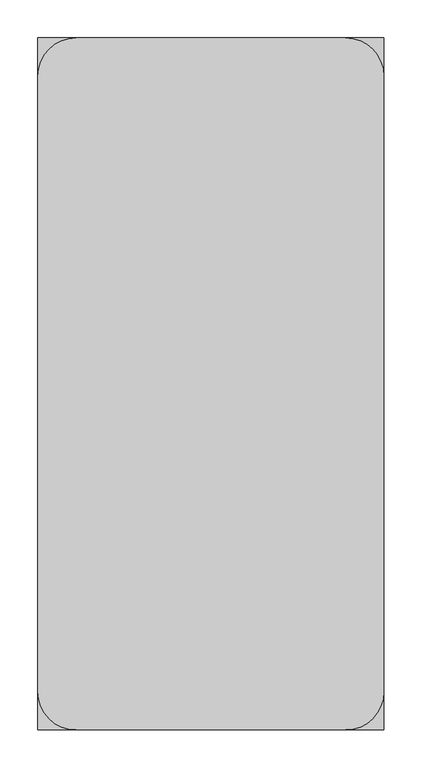
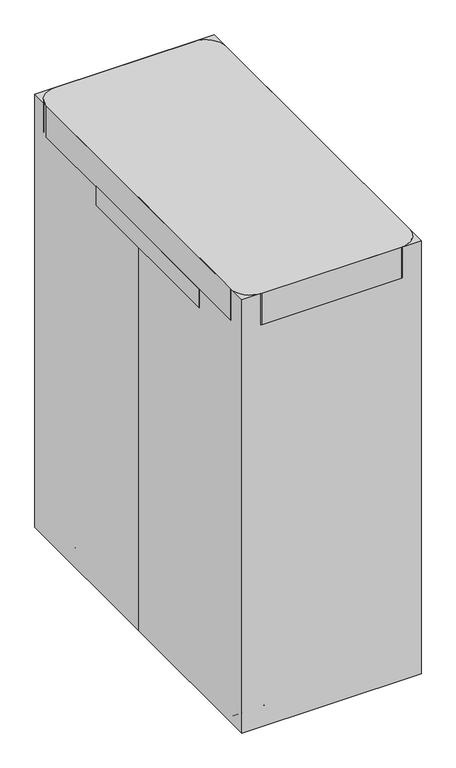
"""IFC4 building model written with IfcOpenShell, lengths in millimetres: proxy geometry, M7040 - Table, Overbed : M7040 - Table, Overbed."""

import ifcopenshell
import ifcopenshell.guid

model = None  # the IFC model being written
_history = None  # IfcOwnerHistory: only IFC2X3 demands one
_inside = {}  # id of a spatial element -> (the spatial element, [elements in it])
_under = {}  # id of a project, library or spatial element -> (it, [spatial elements below it])
_declared = {}  # id of a project -> (the project, [libraries it declares])
_typed = {}  # id of a type object -> (the type object, [elements of that type])
_made_of = {}  # id of a material, layer set ... -> (it, [elements and type objects made of it])


def new_model(schema):
    """Start an empty IFC model of exactly this schema.

    Asked for "IFC4X3", IfcOpenShell would pick the latest addendum, in which some entities
    have other attributes; the version numbers below select the first issue.
    IFC2X3 requires an IfcOwnerHistory on every rooted entity: one is made here for all.
    """
    global model, _history
    if schema == "IFC4X3":
        model = ifcopenshell.file(schema_version=(4, 3, 0, 0))
    else:
        model = ifcopenshell.file(schema=schema)
    _inside.clear()
    _under.clear()
    _declared.clear()
    _typed.clear()
    _made_of.clear()
    _history = None
    if model.schema == "IFC2X3":
        org = make("IfcOrganization", Name="unknown")
        user = make(
            "IfcPersonAndOrganization",
            ThePerson=make("IfcPerson", FamilyName="unknown"),
            TheOrganization=org,
        )
        app = make(
            "IfcApplication",
            ApplicationDeveloper=org,
            Version="unknown",
            ApplicationFullName="unknown",
            ApplicationIdentifier="unknown",
        )
        _history = make(
            "IfcOwnerHistory",
            OwningUser=user,
            OwningApplication=app,
            ChangeAction="ADDED",
            CreationDate=0,
        )
    return model


def make(cls, **values):
    """One entity of the class cls with the attributes given. An attribute that is None is left unset."""
    return model.create_entity(
        cls, **{name: value for name, value in values.items() if value is not None}
    )


def rooted(cls, **values):
    """An entity with a GlobalId (a new one), such as an element, a storey or a relation."""
    return make(cls, GlobalId=ifcopenshell.guid.new(), OwnerHistory=_history, **values)


def si_unit(unit_type, name, prefix=None):
    """IfcSIUnit, for example si_unit("LENGTHUNIT", "METRE", prefix="MILLI")."""
    return make("IfcSIUnit", UnitType=unit_type, Prefix=prefix, Name=name)


def assignment(units):
    """IfcUnitAssignment: the units of a project."""
    return None if units is None else make("IfcUnitAssignment", Units=units)


def point(xyz):
    """IfcCartesianPoint."""
    return None if xyz is None else make("IfcCartesianPoint", Coordinates=xyz)


def direction(xyz):
    """IfcDirection."""
    return None if xyz is None else make("IfcDirection", DirectionRatios=xyz)


def frame(location, z_axis=None, x_axis=None):
    """IfcAxis2Placement3D, a coordinate frame: its origin and axes. An axis left out is left unset."""
    return make(
        "IfcAxis2Placement3D",
        Location=point(location),
        Axis=direction(z_axis),
        RefDirection=direction(x_axis),
    )


def frame_2d(location, x_axis=None):
    """IfcAxis2Placement2D, a coordinate frame in the plane: its origin and x axis."""
    return make(
        "IfcAxis2Placement2D", Location=point(location), RefDirection=direction(x_axis)
    )


def origin():
    """The frame at (0, 0, 0) with its axes left unset."""
    return frame((0.0, 0.0, 0.0))


def origin_with_axes():
    """The frame at (0, 0, 0) with the z axis (0, 0, 1) and the x axis (1, 0, 0) written out."""
    return frame((0.0, 0.0, 0.0), z_axis=(0.0, 0.0, 1.0), x_axis=(1.0, 0.0, 0.0))


def place(relative_to, where):
    """IfcLocalPlacement: puts the frame where relative to a parent placement (None: the world)."""
    return make(
        "IfcLocalPlacement", PlacementRelTo=relative_to, RelativePlacement=where
    )


def context(
    kind, dimensions, precision=None, world=None, true_north=None, identifier=None
):
    """IfcGeometricRepresentationContext, for example the 3D "Model" context."""
    return make(
        "IfcGeometricRepresentationContext",
        ContextIdentifier=identifier,
        ContextType=kind,
        CoordinateSpaceDimension=dimensions,
        Precision=precision,
        WorldCoordinateSystem=world,
        TrueNorth=true_north,
    )


def project(units=None, contexts=None):
    """IfcProject with its units and contexts."""
    return rooted(
        "IfcProject",
        Name="project",
        RepresentationContexts=contexts,
        UnitsInContext=assignment(units),
    )


def spatial(cls, under=None, at=None, **own):
    """A site, building, storey or space (cls), placed at a placement, below another one or the project."""
    s = rooted(cls, ObjectPlacement=at, **own)
    if under is not None:
        _under.setdefault(under.id(), (under, []))[1].append(s)
    return s


def polyline(points):
    """IfcPolyline through the points."""
    return make("IfcPolyline", Points=[point(p) for p in points])


def circle_curve(where, radius):
    """IfcCircle in the frame where."""
    return make("IfcCircle", Position=where, Radius=radius)


def trimmed(basis, trim1, trim2, sense, master):
    """IfcTrimmedCurve: the piece of a basis curve between two trims."""
    return make(
        "IfcTrimmedCurve",
        BasisCurve=basis,
        Trim1=trim1,
        Trim2=trim2,
        SenseAgreement=sense,
        MasterRepresentation=master,
    )


def segment(curve, same_sense, transition):
    """IfcCompositeCurveSegment."""
    return make(
        "IfcCompositeCurveSegment",
        Transition=transition,
        SameSense=same_sense,
        ParentCurve=curve,
    )


def composite_curve(segments, self_intersect=None):
    """IfcCompositeCurve: segments joined end to end."""
    return make("IfcCompositeCurve", Segments=segments, SelfIntersect=self_intersect)


def outline(outer, holes=None, kind="AREA"):
    """IfcArbitraryClosedProfileDef: a profile drawn as a closed curve; with holes, ...WithVoids."""
    if holes is None:
        return make("IfcArbitraryClosedProfileDef", ProfileType=kind, OuterCurve=outer)
    return make(
        "IfcArbitraryProfileDefWithVoids",
        ProfileType=kind,
        OuterCurve=outer,
        InnerCurves=holes,
    )


def extrude(swept, where, along, depth):
    """IfcExtrudedAreaSolid: the profile swept, set in the frame where, extruded along a direction by depth."""
    return make(
        "IfcExtrudedAreaSolid",
        SweptArea=swept,
        Position=where,
        ExtrudedDirection=direction(along),
        Depth=depth,
    )


def shape(context_of_items, identifier, shape_type, items):
    """IfcShapeRepresentation: the items that make up one representation, for example the "Body"."""
    return make(
        "IfcShapeRepresentation",
        ContextOfItems=context_of_items,
        RepresentationIdentifier=identifier,
        RepresentationType=shape_type,
        Items=items,
    )


def source(mapping_origin, context_of_items, identifier, shape_type, items):
    """IfcRepresentationMap: a shape defined once, which mapped items show again and again."""
    return make(
        "IfcRepresentationMap",
        MappingOrigin=mapping_origin,
        MappedRepresentation=shape(context_of_items, identifier, shape_type, items),
    )


def transform(
    local_origin,
    x_axis=None,
    y_axis=None,
    z_axis=None,
    scale=None,
    scale2=None,
    scale3=None,
    uniform=True,
):
    """IfcCartesianTransformationOperator3D, or its non-uniform kind. x_axis, y_axis, z_axis: its Axis1, 2, 3."""
    if uniform:
        return make(
            "IfcCartesianTransformationOperator3D",
            Axis1=direction(x_axis),
            Axis2=direction(y_axis),
            LocalOrigin=point(local_origin),
            Scale=scale,
            Axis3=direction(z_axis),
        )
    return make(
        "IfcCartesianTransformationOperator3DnonUniform",
        Axis1=direction(x_axis),
        Axis2=direction(y_axis),
        LocalOrigin=point(local_origin),
        Scale=scale,
        Axis3=direction(z_axis),
        Scale2=scale2,
        Scale3=scale3,
    )


def mapped(mapping_source, mapping_target):
    """IfcMappedItem: shows the shape of a source again, moved by a transform."""
    return make(
        "IfcMappedItem", MappingSource=mapping_source, MappingTarget=mapping_target
    )


def made_of(thing, what):
    """Note that an element or type object is made of a material, layer set ...; save() writes the relation."""
    if what is not None:
        _made_of.setdefault(what.id(), (what, []))[1].append(thing)
    return thing


def element(
    cls,
    number,
    at=None,
    inside=None,
    cuts=None,
    type_object=None,
    material=None,
    context=None,
    identifier="Body",
    shape_type=None,
    held_by="IfcProductDefinitionShape",
    body=None,
    shapes=None,
    **own,
):
    """One element of the class cls, such as IfcWall. Its Tag is "e" and its number.

    at: its placement. inside: the storey or other place that contains it. cuts: it is an
    opening in that element (IfcRelVoidsElement). A single representation is given by context,
    identifier, shape_type and body (its items); several are given by shapes. held_by: the class
    of the entity that holds the representations. save() writes the other relations.
    """
    e = rooted(cls, Tag="e%d" % number, ObjectPlacement=at, **own)
    if body is not None:
        shapes = [shape(context, identifier, shape_type, body)]
    if shapes is not None:
        e.Representation = make(held_by, Representations=shapes)
    if inside is not None:
        _inside.setdefault(inside.id(), (inside, []))[1].append(e)
    if cuts is not None:
        rooted(
            "IfcRelVoidsElement", RelatingBuildingElement=cuts, RelatedOpeningElement=e
        )
    if type_object is not None:
        _typed.setdefault(type_object.id(), (type_object, []))[1].append(e)
    return made_of(e, material)


def aggregate(whole, parts):
    """IfcRelAggregates: a whole, such as a stair, and the parts it consists of."""
    return rooted("IfcRelAggregates", RelatingObject=whole, RelatedObjects=parts)


def save(model, path):
    """Write the relations noted so far, then the file.

    IfcRelAggregates (storeys below a building ...), IfcRelContainedInSpatialStructure (elements
    in a storey), IfcRelDefinesByType, IfcRelAssociatesMaterial and IfcRelDeclares: one each for
    every whole, place, type object, material and project.
    """
    for whole, parts in _under.values():
        aggregate(whole, parts)
    for where, things in _inside.values():
        rooted(
            "IfcRelContainedInSpatialStructure",
            RelatedElements=things,
            RelatingStructure=where,
        )
    for kind, things in _typed.values():
        rooted("IfcRelDefinesByType", RelatedObjects=things, RelatingType=kind)
    for what, things in _made_of.values():
        rooted("IfcRelAssociatesMaterial", RelatedObjects=things, RelatingMaterial=what)
    for by, libraries in _declared.values():
        rooted("IfcRelDeclares", RelatingContext=by, RelatedDefinitions=libraries)
    model.write(path)


def specialty_equipment_190c61b0(model_context):
    return source(origin(), model_context, "Body", "SweptSolid", [
        extrude(outline(polyline([(228.6, 187.2297287), (228.6, -269.9702713), (-228.6, -269.9702713), (-228.6, 187.2297287), (228.6, 187.2297287)])), frame((0.0, 0.0, 1033.0016667), z_axis=(0.0, 0.0, 1.0), x_axis=(1.0, 0.0, 0.0)), (0.0, 0.0, 1.0), 50.8),
        extrude(outline(polyline([(216.6344082, -319.9060209), (216.6344082, -425.45), (-218.1273098, -425.45), (-218.1273098, -319.9060209), (216.6344082, -319.9060209)])), frame((0.0, 0.0, 127.0), z_axis=(0.0, 0.0, 1.0), x_axis=(1.0, 0.0, 0.0)), (0.0, 0.0, 1.0), 38.1),
        extrude(outline(polyline([(-33.9903673, 310.5535606), (34.925, 310.5535606), (34.925, -319.9060209), (-33.9903673, -319.9060209), (-33.9903673, 310.5535606)])), frame((0.0, 0.0, 127.0), z_axis=(0.0, 0.0, 1.0), x_axis=(1.0, 0.0, 0.0)), (0.0, 0.0, 1.0), 38.1),
        extrude(outline(composite_curve([segment(trimmed(circle_curve(frame_2d((-179.8693101, -389.7056599)), 16.9333333), [point((-196.8026434, -389.7056599))], [point((-162.9359768, -389.7056599))], False, "CARTESIAN"), True, "CONTINUOUS"), segment(trimmed(circle_curve(frame_2d((-179.8693101, -389.7056599)), 16.9333333), [point((-162.9359768, -389.7056599))], [point((-196.8026434, -389.7056599))], False, "CARTESIAN"), True, "CONTINUOUS")], self_intersect=False)), frame((0.0, 0.0, 84.8149176), z_axis=(0.0, 0.0, 1.0), x_axis=(1.0, 0.0, 0.0)), (0.0, 0.0, 1.0), 42.1850824),
        extrude(outline(composite_curve([segment(trimmed(circle_curve(frame_2d((178.8623991, -389.7056599)), 16.9333333), [point((195.7957324, -389.7056599))], [point((161.9290658, -389.7056599))], False, "CARTESIAN"), True, "CONTINUOUS"), segment(trimmed(circle_curve(frame_2d((178.8623991, -389.7056599)), 16.9333333), [point((161.9290658, -389.7056599))], [point((195.7957324, -389.7056599))], False, "CARTESIAN"), True, "CONTINUOUS")], self_intersect=False)), frame((0.0, 0.0, 84.8149176), z_axis=(0.0, 0.0, 1.0), x_axis=(1.0, 0.0, 0.0)), (0.0, 0.0, 1.0), 42.1850824),
        extrude(outline(composite_curve([segment(trimmed(circle_curve(frame_2d((-372.7723265, 50.8)), 50.8), [point((-423.5723265, 50.8))], [point((-321.9723265, 50.8))], False, "CARTESIAN"), True, "CONTINUOUS"), segment(trimmed(circle_curve(frame_2d((-372.7723265, 50.8)), 50.8), [point((-321.9723265, 50.8))], [point((-423.5723265, 50.8))], False, "CARTESIAN"), True, "CONTINUOUS")], self_intersect=False)), frame((140.7840445, 0.0, 0.0), z_axis=(1.0, 0.0, 0.0), x_axis=(0.0, 1.0, 0.0)), (0.0, 0.0, 1.0), 19.05),
        extrude(outline(composite_curve([segment(trimmed(circle_curve(frame_2d((-372.7723265, 50.8)), 50.8), [point((-423.5723265, 50.8))], [point((-321.9723265, 50.8))], False, "CARTESIAN"), True, "CONTINUOUS"), segment(trimmed(circle_curve(frame_2d((-372.7723265, 50.8)), 50.8), [point((-321.9723265, 50.8))], [point((-423.5723265, 50.8))], False, "CARTESIAN"), True, "CONTINUOUS")], self_intersect=False)), frame((197.9340445, 0.0, 0.0), z_axis=(1.0, 0.0, 0.0), x_axis=(0.0, 1.0, 0.0)), (0.0, 0.0, 1.0), 19.05),
        extrude(outline(composite_curve([segment(trimmed(circle_curve(frame_2d((-372.7723265, 50.8)), 33.8666667), [point((-338.9056599, 50.8))], [point((-406.6389932, 50.8))], False, "CARTESIAN"), True, "CONTINUOUS"), segment(trimmed(circle_curve(frame_2d((-372.7723265, 50.8)), 33.8666667), [point((-406.6389932, 50.8))], [point((-338.9056599, 50.8))], False, "CARTESIAN"), True, "CONTINUOUS")], self_intersect=False)), frame((159.8340445, 0.0, 0.0), z_axis=(1.0, 0.0, 0.0), x_axis=(0.0, 1.0, 0.0)), (0.0, 0.0, 1.0), 38.1),
        extrude(outline(composite_curve([segment(trimmed(circle_curve(frame_2d((-372.7723265, 50.8)), 50.8), [point((-423.5723265, 50.8))], [point((-321.9723265, 50.8))], False, "CARTESIAN"), True, "CONTINUOUS"), segment(trimmed(circle_curve(frame_2d((-372.7723265, 50.8)), 50.8), [point((-321.9723265, 50.8))], [point((-423.5723265, 50.8))], False, "CARTESIAN"), True, "CONTINUOUS")], self_intersect=False)), frame((-160.6276735, 0.0, 0.0), z_axis=(1.0, 0.0, 0.0), x_axis=(0.0, 1.0, 0.0)), (0.0, 0.0, 1.0), 19.05),
        extrude(outline(composite_curve([segment(trimmed(circle_curve(frame_2d((-372.7723265, 50.8)), 50.8), [point((-423.5723265, 50.8))], [point((-321.9723265, 50.8))], False, "CARTESIAN"), True, "CONTINUOUS"), segment(trimmed(circle_curve(frame_2d((-372.7723265, 50.8)), 50.8), [point((-321.9723265, 50.8))], [point((-423.5723265, 50.8))], False, "CARTESIAN"), True, "CONTINUOUS")], self_intersect=False)), frame((-217.7776735, 0.0, 0.0), z_axis=(1.0, 0.0, 0.0), x_axis=(0.0, 1.0, 0.0)), (0.0, 0.0, 1.0), 19.05),
        extrude(outline(composite_curve([segment(trimmed(circle_curve(frame_2d((-372.7723265, 50.8)), 33.8666667), [point((-338.9056599, 50.8))], [point((-406.6389932, 50.8))], False, "CARTESIAN"), True, "CONTINUOUS"), segment(trimmed(circle_curve(frame_2d((-372.7723265, 50.8)), 33.8666667), [point((-406.6389932, 50.8))], [point((-338.9056599, 50.8))], False, "CARTESIAN"), True, "CONTINUOUS")], self_intersect=False)), frame((-198.7276735, 0.0, 0.0), z_axis=(1.0, 0.0, 0.0), x_axis=(0.0, 1.0, 0.0)), (0.0, 0.0, 1.0), 38.1),
        extrude(outline(composite_curve([segment(trimmed(circle_curve(frame_2d((-180.2189464, 378.2868939)), 16.9333333), [point((-197.1522798, 378.2868939))], [point((-163.2856131, 378.2868939))], False, "CARTESIAN"), True, "CONTINUOUS"), segment(trimmed(circle_curve(frame_2d((-180.2189464, 378.2868939)), 16.9333333), [point((-163.2856131, 378.2868939))], [point((-197.1522798, 378.2868939))], False, "CARTESIAN"), True, "CONTINUOUS")], self_intersect=False)), frame((0.0, 0.0, 84.8149176), z_axis=(0.0, 0.0, 1.0), x_axis=(1.0, 0.0, 0.0)), (0.0, 0.0, 1.0), 42.1850824),
        extrude(outline(composite_curve([segment(trimmed(circle_curve(frame_2d((178.5127627, 378.2868939)), 16.9333333), [point((195.4460961, 378.2868939))], [point((161.5794294, 378.2868939))], False, "CARTESIAN"), True, "CONTINUOUS"), segment(trimmed(circle_curve(frame_2d((178.5127627, 378.2868939)), 16.9333333), [point((161.5794294, 378.2868939))], [point((195.4460961, 378.2868939))], False, "CARTESIAN"), True, "CONTINUOUS")], self_intersect=False)), frame((0.0, 0.0, 84.8149176), z_axis=(0.0, 0.0, 1.0), x_axis=(1.0, 0.0, 0.0)), (0.0, 0.0, 1.0), 42.1850824),
        extrude(outline(composite_curve([segment(trimmed(circle_curve(frame_2d((361.3535606, 50.8)), 50.8), [point((412.1535606, 50.8))], [point((310.5535606, 50.8))], False, "CARTESIAN"), True, "CONTINUOUS"), segment(trimmed(circle_curve(frame_2d((361.3535606, 50.8)), 50.8), [point((310.5535606, 50.8))], [point((412.1535606, 50.8))], False, "CARTESIAN"), True, "CONTINUOUS")], self_intersect=False)), frame((140.4344082, 0.0, 0.0), z_axis=(1.0, 0.0, 0.0), x_axis=(0.0, 1.0, 0.0)), (0.0, 0.0, 1.0), 19.05),
        extrude(outline(composite_curve([segment(trimmed(circle_curve(frame_2d((361.3535606, 50.8)), 50.8), [point((412.1535606, 50.8))], [point((310.5535606, 50.8))], False, "CARTESIAN"), True, "CONTINUOUS"), segment(trimmed(circle_curve(frame_2d((361.3535606, 50.8)), 50.8), [point((310.5535606, 50.8))], [point((412.1535606, 50.8))], False, "CARTESIAN"), True, "CONTINUOUS")], self_intersect=False)), frame((197.5844082, 0.0, 0.0), z_axis=(1.0, 0.0, 0.0), x_axis=(0.0, 1.0, 0.0)), (0.0, 0.0, 1.0), 19.05),
        extrude(outline(composite_curve([segment(trimmed(circle_curve(frame_2d((361.3535606, 50.8)), 33.8666667), [point((327.4868939, 50.8))], [point((395.2202273, 50.8))], False, "CARTESIAN"), True, "CONTINUOUS"), segment(trimmed(circle_curve(frame_2d((361.3535606, 50.8)), 33.8666667), [point((395.2202273, 50.8))], [point((327.4868939, 50.8))], False, "CARTESIAN"), True, "CONTINUOUS")], self_intersect=False)), frame((159.4844082, 0.0, 0.0), z_axis=(1.0, 0.0, 0.0), x_axis=(0.0, 1.0, 0.0)), (0.0, 0.0, 1.0), 38.1),
        extrude(outline(composite_curve([segment(trimmed(circle_curve(frame_2d((361.3535606, 50.8)), 50.8), [point((412.1535606, 50.8))], [point((310.5535606, 50.8))], False, "CARTESIAN"), True, "CONTINUOUS"), segment(trimmed(circle_curve(frame_2d((361.3535606, 50.8)), 50.8), [point((310.5535606, 50.8))], [point((412.1535606, 50.8))], False, "CARTESIAN"), True, "CONTINUOUS")], self_intersect=False)), frame((-160.9773098, 0.0, 0.0), z_axis=(1.0, 0.0, 0.0), x_axis=(0.0, 1.0, 0.0)), (0.0, 0.0, 1.0), 19.05),
        extrude(outline(composite_curve([segment(trimmed(circle_curve(frame_2d((361.3535606, 50.8)), 50.8), [point((412.1535606, 50.8))], [point((310.5535606, 50.8))], False, "CARTESIAN"), True, "CONTINUOUS"), segment(trimmed(circle_curve(frame_2d((361.3535606, 50.8)), 50.8), [point((310.5535606, 50.8))], [point((412.1535606, 50.8))], False, "CARTESIAN"), True, "CONTINUOUS")], self_intersect=False)), frame((-218.1273098, 0.0, 0.0), z_axis=(1.0, 0.0, 0.0), x_axis=(0.0, 1.0, 0.0)), (0.0, 0.0, 1.0), 19.05),
        extrude(outline(composite_curve([segment(trimmed(circle_curve(frame_2d((361.3535606, 50.8)), 33.8666667), [point((327.4868939, 50.8))], [point((395.2202273, 50.8))], False, "CARTESIAN"), True, "CONTINUOUS"), segment(trimmed(circle_curve(frame_2d((361.3535606, 50.8)), 33.8666667), [point((395.2202273, 50.8))], [point((327.4868939, 50.8))], False, "CARTESIAN"), True, "CONTINUOUS")], self_intersect=False)), frame((-199.0773098, 0.0, 0.0), z_axis=(1.0, 0.0, 0.0), x_axis=(0.0, 1.0, 0.0)), (0.0, 0.0, 1.0), 38.1),
        extrude(outline(polyline([(216.6344082, 446.8913935), (216.6344082, 310.5535606), (-218.1273098, 310.5535606), (-218.1273098, 446.8913935), (216.6344082, 446.8913935)])), frame((0.0, 0.0, 127.0), z_axis=(0.0, 0.0, 1.0), x_axis=(1.0, 0.0, 0.0)), (0.0, 0.0, 1.0), 38.1),
        extrude(outline(polyline([(44.45, 424.8535606), (44.45, 335.9535606), (-44.45, 335.9535606), (-44.45, 424.8535606), (44.45, 424.8535606)])), frame((0.0, 0.0, 165.1), z_axis=(0.0, 0.0, 1.0), x_axis=(1.0, 0.0, 0.0)), (0.0, 0.0, 1.0), 258.3016667),
        extrude(outline(polyline([(50.8, 431.2035606), (50.8, 329.6035606), (-50.8, 329.6035606), (-50.8, 431.2035606), (50.8, 431.2035606)])), frame((0.0, 0.0, 423.4016667), z_axis=(0.0, 0.0, 1.0), x_axis=(1.0, 0.0, 0.0)), (0.0, 0.0, 1.0), 660.4),
        extrude(outline(composite_curve([segment(trimmed(circle_curve(frame_2d((-177.8, 406.4)), 50.8), [point((-228.6, 406.4))], [point((-177.8, 457.2))], False, "CARTESIAN"), True, "CONTINUOUS"), segment(polyline([(-177.8, 457.2), (177.8, 457.2)]), True, "CONTINUOUS"), segment(trimmed(circle_curve(frame_2d((177.8, 406.4)), 50.8), [point((177.8, 457.2))], [point((228.6, 406.4))], False, "CARTESIAN"), True, "CONTINUOUS"), segment(polyline([(228.6, 406.4), (228.6, -406.4)]), True, "CONTINUOUS"), segment(trimmed(circle_curve(frame_2d((177.8, -406.4)), 50.8), [point((228.6, -406.4))], [point((177.8, -457.2))], False, "CARTESIAN"), True, "CONTINUOUS"), segment(polyline([(177.8, -457.2), (-177.8, -457.2)]), True, "CONTINUOUS"), segment(trimmed(circle_curve(frame_2d((-177.8, -406.4)), 50.8), [point((-177.8, -457.2))], [point((-228.6, -406.4))], False, "CARTESIAN"), True, "CONTINUOUS"), segment(polyline([(-228.6, -406.4), (-228.6, 406.4)]), True, "CONTINUOUS")], self_intersect=False)), frame((0.0, 0.0, 1083.8016667), z_axis=(0.0, 0.0, 1.0), x_axis=(1.0, 0.0, 0.0)), (0.0, 0.0, 1.0), 84.5983333),
        extrude(outline(polyline([(-228.6, 457.2), (228.6, 457.2), (228.6, -457.2), (-228.6, -457.2), (-228.6, 0.0), (-228.6, 457.2)])), origin_with_axes(), (0.0, 0.0, 1.0), 1168.4),
    ])


if __name__ == "__main__":
    model = new_model("IFC4")
    model_context = context("Model", 3, world=origin())
    ifc_project = project(units=[si_unit("LENGTHUNIT", "METRE", prefix="MILLI")], contexts=[model_context])
    site = spatial("IfcSite", under=ifc_project)
    building = spatial("IfcBuilding", under=site)
    placement = place(None, origin())
    specialty_equipment_shape = specialty_equipment_190c61b0(model_context)
    element("IfcBuildingElementProxy", 1, Name="M7040 - Table, Overbed : M7040 - Table, Overbed", ObjectType="M7040 - Table, Overbed : M7040 - Table, Overbed", at=placement, inside=building, context=model_context, shape_type="MappedRepresentation", body=[
        mapped(specialty_equipment_shape, transform((0.0, 0.0, 0.0), x_axis=(1.0, 0.0, 0.0), y_axis=(0.0, 1.0, 0.0), z_axis=(0.0, 0.0, 1.0))),
    ])
    save(model, "model.ifc")

# Revit data of these elements
# Type "M7040 - Table, Overbed : M7040 - Table, Overbed"
#   Watts2 = "0"
#   Watts1 = "0"
#   Unit_Issue = "EA"
#   UTIL_6_Misc = "-"
#   UTIL_5_NonMedGas = "-"
#   UTIL_4_MiscGas = "-"
#   UTIL_3_MedGas = "-"
#   UTIL_2_Elec = "-"
#   UTIL_1_WaterDrain = "-"
#   Nomenclature = "Table, Overbed"
#   NSN = "6515"
#   Location [instance default] = ""
#   JSN = "M7040"
#   Fund_Source_VA = "-"
#   Fund_Source_Navy = "-"
#   Fund_Source_Army = "-"
#   Fund_Source_AF = "-"
#   ELEC_Volts2 = "0"
#   ELEC_Volts1 = "0"
#   ELEC_Phase2 = "0"
#   ELEC_Phase1 = "0"
#   ELEC_HertzSwitch = "0"
#   ELEC_HertzDependent = "0"
#   ELEC_Hertz = "0"
#   ELEC_Amps2 = "0"
#   ELEC_Amps1 = "0"
#   DetailDescription = "Overbed table. Adjustable height table constructed of heavy gauge steel. Mounted on 2\" diameter twin swivel casters with bumper caps. Table top is constructed with a high pressure plastic laminated surface that resists chipping, scratching, and staining. It includes a vanity tray and a mirror. Table is designed for use over bed, wheelchair or large chair."
#   CAT_VA = "C"
#   CAT_Navy = "C"
#   CAT_IHS = "-"
#   CAT_Army = "C"
#   CAT_AF = "C"
#   BTUperhour = "0"
#   radius = 0' - 2"
#   calc 2 = 0' - 0.66667"
#   calc 1 = 0' - 1.33333"
#   Weight_IP = 50
#   DIM_Width_IP = 1' - 6"
#   DIM_Height_IP = 3' - 10"
#   DIM_Depth_IP = 3' - 0"
#   top [instance default] = none
#   finish [instance default] = none
# Element 1 (IfcBuildingElementProxy, "M7040 - Table, Overbed : M7040 - Table, Overbed")
#   Location = "BRMS1"
#   Materials on its faces: "EquipSpace"
# Materials
#   "EquipSpace": class "Unassigned", colour RGB 221 217 195, transparency 0.5
